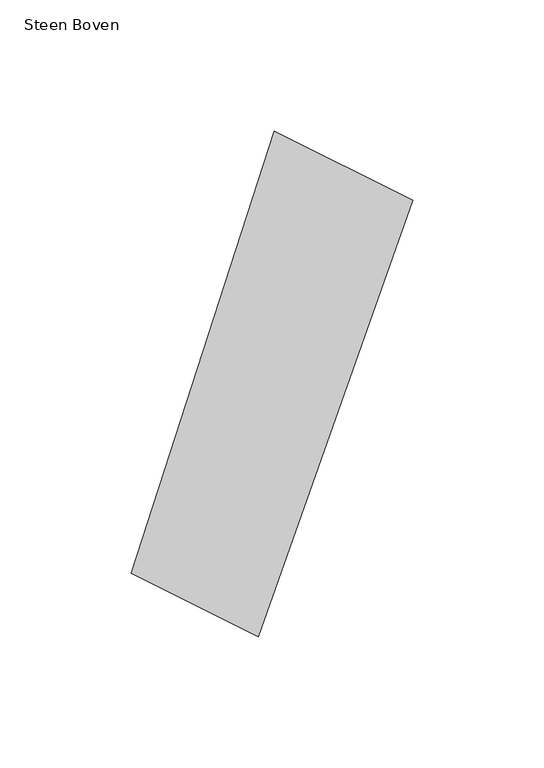
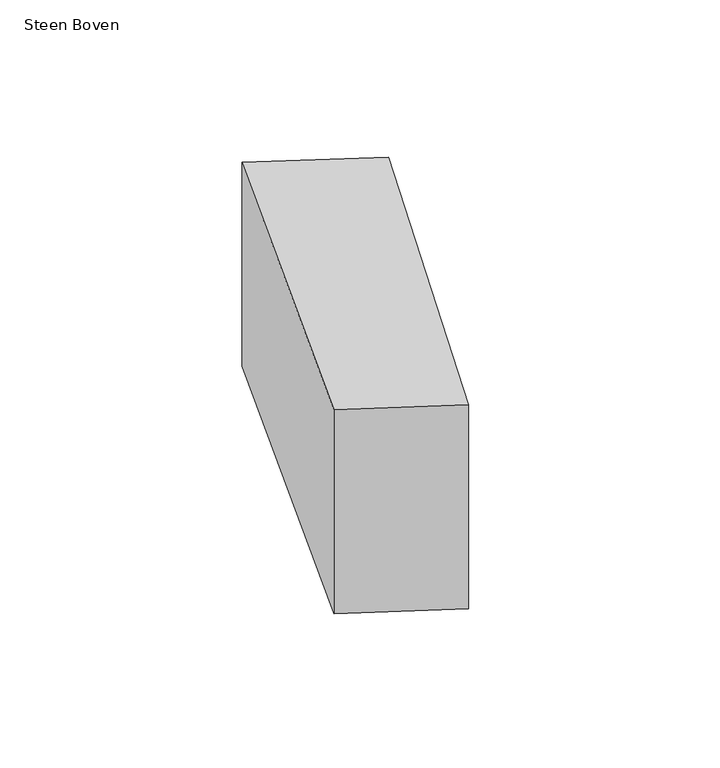
"""IFC4 building model written with IfcOpenShell, lengths in millimetres: proxy geometry, 00_GMA_steen_versie_4 : Steen Boven."""

from ifc_helpers import new_model, si_unit, origin, origin_with_axes, place, context, project, spatial, polyline, outline, extrude, source, transform, mapped, element, save


def steen_boven_bf928b71(model_context):
    return source(origin(), model_context, "Body", "SweptSolid", [
        extrude(outline(polyline([(131.3439546, 156.325315), (72.4861881, -9.947783), (24.062053, 14.2514216), (78.6055909, 182.699492), (131.3439546, 156.325315)])), origin_with_axes(), (0.0, 0.0, 1.0), 100.0),
    ])


if __name__ == "__main__":
    model = new_model("IFC4")
    model_context = context("Model", 3, world=origin())
    ifc_project = project(units=[si_unit("LENGTHUNIT", "METRE", prefix="MILLI")], contexts=[model_context])
    site = spatial("IfcSite", under=ifc_project)
    building = spatial("IfcBuilding", under=site)
    placement = place(None, origin())
    steen_boven_shape = steen_boven_bf928b71(model_context)
    element("IfcBuildingElementProxy", 1, Name="00_GMA_steen_versie_4 : Steen Boven", ObjectType="00_GMA_steen_versie_4 : Steen Boven", at=placement, inside=building, context=model_context, shape_type="MappedRepresentation", body=[
        mapped(steen_boven_shape, transform((0.0, 0.0, 0.0), x_axis=(1.0, 0.0, 0.0), y_axis=(0.0, 1.0, 0.0), z_axis=(0.0, 0.0, 1.0))),
    ])
    save(model, "model.ifc")

# Revit data of these elements
# Type "00_GMA_steen_versie_4 : Steen Boven"
#   StootVoegHalfBoven [instance default] = 5 mm
#   StootVoegHalf [instance default] = 5 mm
#   StootVoegBreedteOnder = 10 mm
#   StootVoegBreedteBoven = 10 mm
#   Steendikte = 100 mm
#   LintVoegOnderHalf = 5 mm
#   LintVoegOnder = 10 mm
#   LintVoegBovenHalf = 0 mm
#   LintVoegBoven = 0 mm
#   materiaal = none
#   MateriaalVoeg = none
#   Default Elevation = 0
